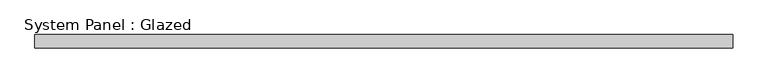
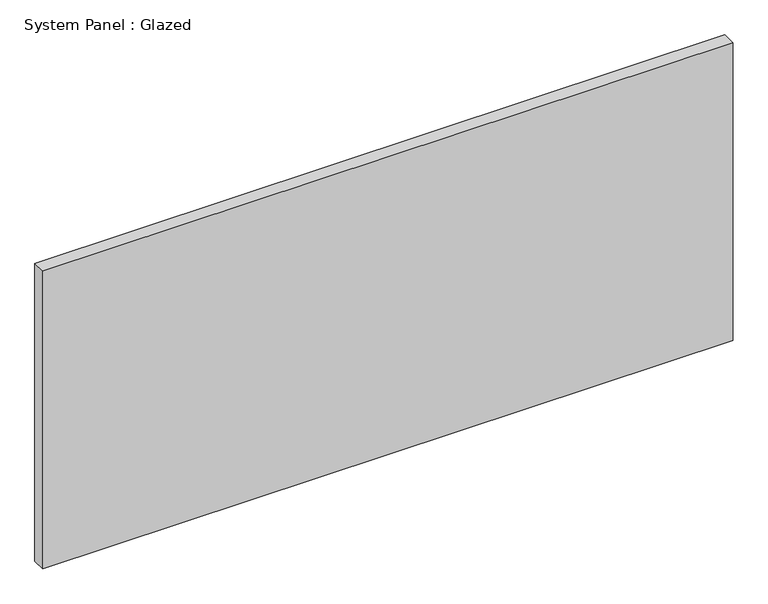
"""IFC4 building model written with IfcOpenShell, lengths in millimetres: plate geometry, System Panel : Glazed."""

import ifcopenshell
import ifcopenshell.guid

model = None  # the IFC model being written
_history = None  # IfcOwnerHistory: only IFC2X3 demands one
_inside = {}  # id of a spatial element -> (the spatial element, [elements in it])
_under = {}  # id of a project, library or spatial element -> (it, [spatial elements below it])
_declared = {}  # id of a project -> (the project, [libraries it declares])
_typed = {}  # id of a type object -> (the type object, [elements of that type])
_made_of = {}  # id of a material, layer set ... -> (it, [elements and type objects made of it])


def new_model(schema):
    """Start an empty IFC model of exactly this schema.

    Asked for "IFC4X3", IfcOpenShell would pick the latest addendum, in which some entities
    have other attributes; the version numbers below select the first issue.
    IFC2X3 requires an IfcOwnerHistory on every rooted entity: one is made here for all.
    """
    global model, _history
    if schema == "IFC4X3":
        model = ifcopenshell.file(schema_version=(4, 3, 0, 0))
    else:
        model = ifcopenshell.file(schema=schema)
    _inside.clear()
    _under.clear()
    _declared.clear()
    _typed.clear()
    _made_of.clear()
    _history = None
    if model.schema == "IFC2X3":
        org = make("IfcOrganization", Name="unknown")
        user = make(
            "IfcPersonAndOrganization",
            ThePerson=make("IfcPerson", FamilyName="unknown"),
            TheOrganization=org,
        )
        app = make(
            "IfcApplication",
            ApplicationDeveloper=org,
            Version="unknown",
            ApplicationFullName="unknown",
            ApplicationIdentifier="unknown",
        )
        _history = make(
            "IfcOwnerHistory",
            OwningUser=user,
            OwningApplication=app,
            ChangeAction="ADDED",
            CreationDate=0,
        )
    return model


def make(cls, **values):
    """One entity of the class cls with the attributes given. An attribute that is None is left unset."""
    return model.create_entity(
        cls, **{name: value for name, value in values.items() if value is not None}
    )


def rooted(cls, **values):
    """An entity with a GlobalId (a new one), such as an element, a storey or a relation."""
    return make(cls, GlobalId=ifcopenshell.guid.new(), OwnerHistory=_history, **values)


def si_unit(unit_type, name, prefix=None):
    """IfcSIUnit, for example si_unit("LENGTHUNIT", "METRE", prefix="MILLI")."""
    return make("IfcSIUnit", UnitType=unit_type, Prefix=prefix, Name=name)


def assignment(units):
    """IfcUnitAssignment: the units of a project."""
    return None if units is None else make("IfcUnitAssignment", Units=units)


def point(xyz):
    """IfcCartesianPoint."""
    return None if xyz is None else make("IfcCartesianPoint", Coordinates=xyz)


def direction(xyz):
    """IfcDirection."""
    return None if xyz is None else make("IfcDirection", DirectionRatios=xyz)


def frame(location, z_axis=None, x_axis=None):
    """IfcAxis2Placement3D, a coordinate frame: its origin and axes. An axis left out is left unset."""
    return make(
        "IfcAxis2Placement3D",
        Location=point(location),
        Axis=direction(z_axis),
        RefDirection=direction(x_axis),
    )


def origin():
    """The frame at (0, 0, 0) with its axes left unset."""
    return frame((0.0, 0.0, 0.0))


def origin_with_axes():
    """The frame at (0, 0, 0) with the z axis (0, 0, 1) and the x axis (1, 0, 0) written out."""
    return frame((0.0, 0.0, 0.0), z_axis=(0.0, 0.0, 1.0), x_axis=(1.0, 0.0, 0.0))


def place(relative_to, where):
    """IfcLocalPlacement: puts the frame where relative to a parent placement (None: the world)."""
    return make(
        "IfcLocalPlacement", PlacementRelTo=relative_to, RelativePlacement=where
    )


def context(
    kind, dimensions, precision=None, world=None, true_north=None, identifier=None
):
    """IfcGeometricRepresentationContext, for example the 3D "Model" context."""
    return make(
        "IfcGeometricRepresentationContext",
        ContextIdentifier=identifier,
        ContextType=kind,
        CoordinateSpaceDimension=dimensions,
        Precision=precision,
        WorldCoordinateSystem=world,
        TrueNorth=true_north,
    )


def project(units=None, contexts=None):
    """IfcProject with its units and contexts."""
    return rooted(
        "IfcProject",
        Name="project",
        RepresentationContexts=contexts,
        UnitsInContext=assignment(units),
    )


def spatial(cls, under=None, at=None, **own):
    """A site, building, storey or space (cls), placed at a placement, below another one or the project."""
    s = rooted(cls, ObjectPlacement=at, **own)
    if under is not None:
        _under.setdefault(under.id(), (under, []))[1].append(s)
    return s


def polyline(points):
    """IfcPolyline through the points."""
    return make("IfcPolyline", Points=[point(p) for p in points])


def outline(outer, holes=None, kind="AREA"):
    """IfcArbitraryClosedProfileDef: a profile drawn as a closed curve; with holes, ...WithVoids."""
    if holes is None:
        return make("IfcArbitraryClosedProfileDef", ProfileType=kind, OuterCurve=outer)
    return make(
        "IfcArbitraryProfileDefWithVoids",
        ProfileType=kind,
        OuterCurve=outer,
        InnerCurves=holes,
    )


def extrude(swept, where, along, depth):
    """IfcExtrudedAreaSolid: the profile swept, set in the frame where, extruded along a direction by depth."""
    return make(
        "IfcExtrudedAreaSolid",
        SweptArea=swept,
        Position=where,
        ExtrudedDirection=direction(along),
        Depth=depth,
    )


def shape(context_of_items, identifier, shape_type, items):
    """IfcShapeRepresentation: the items that make up one representation, for example the "Body"."""
    return make(
        "IfcShapeRepresentation",
        ContextOfItems=context_of_items,
        RepresentationIdentifier=identifier,
        RepresentationType=shape_type,
        Items=items,
    )


def source(mapping_origin, context_of_items, identifier, shape_type, items):
    """IfcRepresentationMap: a shape defined once, which mapped items show again and again."""
    return make(
        "IfcRepresentationMap",
        MappingOrigin=mapping_origin,
        MappedRepresentation=shape(context_of_items, identifier, shape_type, items),
    )


def transform(
    local_origin,
    x_axis=None,
    y_axis=None,
    z_axis=None,
    scale=None,
    scale2=None,
    scale3=None,
    uniform=True,
):
    """IfcCartesianTransformationOperator3D, or its non-uniform kind. x_axis, y_axis, z_axis: its Axis1, 2, 3."""
    if uniform:
        return make(
            "IfcCartesianTransformationOperator3D",
            Axis1=direction(x_axis),
            Axis2=direction(y_axis),
            LocalOrigin=point(local_origin),
            Scale=scale,
            Axis3=direction(z_axis),
        )
    return make(
        "IfcCartesianTransformationOperator3DnonUniform",
        Axis1=direction(x_axis),
        Axis2=direction(y_axis),
        LocalOrigin=point(local_origin),
        Scale=scale,
        Axis3=direction(z_axis),
        Scale2=scale2,
        Scale3=scale3,
    )


def mapped(mapping_source, mapping_target):
    """IfcMappedItem: shows the shape of a source again, moved by a transform."""
    return make(
        "IfcMappedItem", MappingSource=mapping_source, MappingTarget=mapping_target
    )


def made_of(thing, what):
    """Note that an element or type object is made of a material, layer set ...; save() writes the relation."""
    if what is not None:
        _made_of.setdefault(what.id(), (what, []))[1].append(thing)
    return thing


def element(
    cls,
    number,
    at=None,
    inside=None,
    cuts=None,
    type_object=None,
    material=None,
    context=None,
    identifier="Body",
    shape_type=None,
    held_by="IfcProductDefinitionShape",
    body=None,
    shapes=None,
    **own,
):
    """One element of the class cls, such as IfcWall. Its Tag is "e" and its number.

    at: its placement. inside: the storey or other place that contains it. cuts: it is an
    opening in that element (IfcRelVoidsElement). A single representation is given by context,
    identifier, shape_type and body (its items); several are given by shapes. held_by: the class
    of the entity that holds the representations. save() writes the other relations.
    """
    e = rooted(cls, Tag="e%d" % number, ObjectPlacement=at, **own)
    if body is not None:
        shapes = [shape(context, identifier, shape_type, body)]
    if shapes is not None:
        e.Representation = make(held_by, Representations=shapes)
    if inside is not None:
        _inside.setdefault(inside.id(), (inside, []))[1].append(e)
    if cuts is not None:
        rooted(
            "IfcRelVoidsElement", RelatingBuildingElement=cuts, RelatedOpeningElement=e
        )
    if type_object is not None:
        _typed.setdefault(type_object.id(), (type_object, []))[1].append(e)
    return made_of(e, material)


def aggregate(whole, parts):
    """IfcRelAggregates: a whole, such as a stair, and the parts it consists of."""
    return rooted("IfcRelAggregates", RelatingObject=whole, RelatedObjects=parts)


def save(model, path):
    """Write the relations noted so far, then the file.

    IfcRelAggregates (storeys below a building ...), IfcRelContainedInSpatialStructure (elements
    in a storey), IfcRelDefinesByType, IfcRelAssociatesMaterial and IfcRelDeclares: one each for
    every whole, place, type object, material and project.
    """
    for whole, parts in _under.values():
        aggregate(whole, parts)
    for where, things in _inside.values():
        rooted(
            "IfcRelContainedInSpatialStructure",
            RelatedElements=things,
            RelatingStructure=where,
        )
    for kind, things in _typed.values():
        rooted("IfcRelDefinesByType", RelatedObjects=things, RelatingType=kind)
    for what, things in _made_of.values():
        rooted("IfcRelAssociatesMaterial", RelatedObjects=things, RelatingMaterial=what)
    for by, libraries in _declared.values():
        rooted("IfcRelDeclares", RelatingContext=by, RelatedDefinitions=libraries)
    model.write(path)


def system_panel_glazed_6728f955(model_context):
    return source(origin(), model_context, "Body", "SweptSolid", [
        extrude(outline(polyline([(654.05, 19.05), (-654.05, 19.05), (-654.05, 44.45), (654.05, 44.45), (654.05, 19.05)])), origin_with_axes(), (0.0, 0.0, 1.0), 596.9),
    ])


if __name__ == "__main__":
    model = new_model("IFC4")
    model_context = context("Model", 3, world=origin())
    ifc_project = project(units=[si_unit("LENGTHUNIT", "METRE", prefix="MILLI")], contexts=[model_context])
    site = spatial("IfcSite", under=ifc_project)
    building = spatial("IfcBuilding", under=site)
    placement = place(None, origin())
    system_panel_glazed_shape = system_panel_glazed_6728f955(model_context)
    element("IfcPlate", 1, ObjectType="System Panel : Glazed", at=placement, inside=building, context=model_context, shape_type="MappedRepresentation", body=[
        mapped(system_panel_glazed_shape, transform((0.0, 0.0, 0.0), x_axis=(1.0, 0.0, 0.0), y_axis=(0.0, 1.0, 0.0), z_axis=(0.0, 0.0, 1.0))),
    ])
    save(model, "model.ifc")

# Revit data of these elements
# Element 1 (IfcPlate, "System Panel : Glazed")
#   Materials on its faces: "Glass"
# Materials
#   "Glass": class "Glass", colour RGB 0 128 192, transparency 0.75
